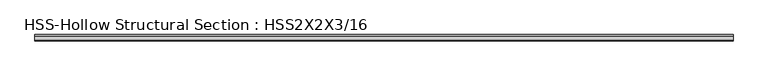
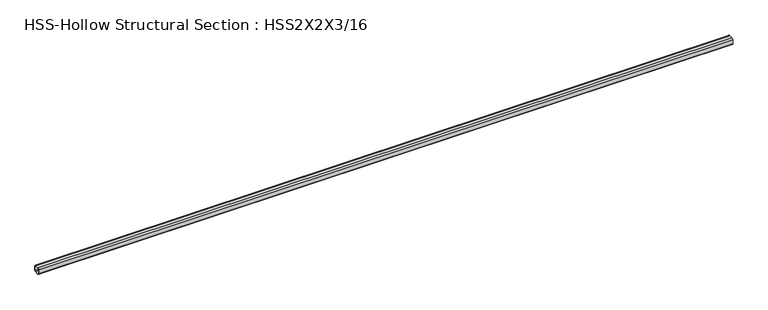
"""IFC4 building model written with IfcOpenShell, lengths in millimetres: beam geometry, HSS-Hollow Structural Section : HSS2X2X3/16."""

from ifc_helpers import new_model, si_unit, point, frame, frame_2d, origin, place, context, project, spatial, polyline, circle_curve, trimmed, segment, composite_curve, outline, extrude, source, transform, mapped, element, save


def hss_hollow_structural_section_hss2x2x3_16_21cd95f6(model_context):
    return source(origin(), model_context, "Body", "SweptSolid", [
        extrude(outline(composite_curve([segment(polyline([(25.4, 16.5608), (25.4, -16.5608)]), True, "CONTINUOUS"), segment(trimmed(circle_curve(frame_2d((16.5608, -16.5608)), 8.8392), [point((25.4, -16.5608))], [point((16.5608, -25.4))], False, "CARTESIAN"), True, "CONTINUOUS"), segment(polyline([(16.5608, -25.4), (-16.5608, -25.4)]), True, "CONTINUOUS"), segment(trimmed(circle_curve(frame_2d((-16.5608, -16.5608)), 8.8392), [point((-16.5608, -25.4))], [point((-25.4, -16.5608))], False, "CARTESIAN"), True, "CONTINUOUS"), segment(polyline([(-25.4, -16.5608), (-25.4, 16.5608)]), True, "CONTINUOUS"), segment(trimmed(circle_curve(frame_2d((-16.5608, 16.5608)), 8.8392), [point((-25.4, 16.5608))], [point((-16.5608, 25.4))], False, "CARTESIAN"), True, "CONTINUOUS"), segment(polyline([(-16.5608, 25.4), (16.5608, 25.4)]), True, "CONTINUOUS"), segment(trimmed(circle_curve(frame_2d((16.5608, 16.5608)), 8.8392), [point((16.5608, 25.4))], [point((25.4, 16.5608))], False, "CARTESIAN"), True, "CONTINUOUS")], self_intersect=False), holes=[composite_curve([segment(trimmed(circle_curve(frame_2d((-16.5608, 16.5608)), 4.4196), [point((-16.5608, 20.9804))], [point((-20.9804, 16.5608))], True, "CARTESIAN"), True, "CONTINUOUS"), segment(polyline([(-20.9804, 16.5608), (-20.9804, -16.5608)]), True, "CONTINUOUS"), segment(trimmed(circle_curve(frame_2d((-16.5608, -16.5608)), 4.4196), [point((-20.9804, -16.5608))], [point((-16.5608, -20.9804))], True, "CARTESIAN"), True, "CONTINUOUS"), segment(polyline([(-16.5608, -20.9804), (16.5608, -20.9804)]), True, "CONTINUOUS"), segment(trimmed(circle_curve(frame_2d((16.5608, -16.5608)), 4.4196), [point((16.5608, -20.9804))], [point((20.9804, -16.5608))], True, "CARTESIAN"), True, "CONTINUOUS"), segment(polyline([(20.9804, -16.5608), (20.9804, 16.5608)]), True, "CONTINUOUS"), segment(trimmed(circle_curve(frame_2d((16.5608, 16.5608)), 4.4196), [point((20.9804, 16.5608))], [point((16.5608, 20.9804))], True, "CARTESIAN"), True, "CONTINUOUS"), segment(polyline([(16.5608, 20.9804), (-16.5608, 20.9804)]), True, "CONTINUOUS")], self_intersect=False)]), frame((4003.675, 0.0, 0.0), z_axis=(1.0, 0.0, 0.0), x_axis=(0.0, 1.0, 0.0)), (0.0, 0.0, 1.0), 5458.61875),
    ])


if __name__ == "__main__":
    model = new_model("IFC4")
    model_context = context("Model", 3, world=origin())
    ifc_project = project(units=[si_unit("LENGTHUNIT", "METRE", prefix="MILLI")], contexts=[model_context])
    site = spatial("IfcSite", under=ifc_project)
    building = spatial("IfcBuilding", under=site)
    placement = place(None, origin())
    hss_hollow_structural_section_hss2x2x3_16_shape = hss_hollow_structural_section_hss2x2x3_16_21cd95f6(model_context)
    element("IfcBeam", 1, ObjectType="HSS-Hollow Structural Section : HSS2X2X3/16", at=placement, inside=building, context=model_context, shape_type="MappedRepresentation", body=[
        mapped(hss_hollow_structural_section_hss2x2x3_16_shape, transform((0.0, 0.0, 0.0), x_axis=(1.0, 0.0, 0.0), y_axis=(0.0, 1.0, 0.0), z_axis=(0.0, 0.0, 1.0))),
    ])
    save(model, "model.ifc")

# Revit data of these elements
# Type "HSS-Hollow Structural Section : HSS2X2X3/16"
#   Keynote = "M05121300.04"
#   Assembly Code = "B10"
#   Shape = "Square"
#   W = 4.3
#   Ht = 0' - 2"
#   Length [instance default] = 5' - 0"
#   b = 0' - 2"
#   kr = 0' - 0.348"
#   t = 0' - 0.174"
#   A = 0.00826389 SF
#   Structural Material [instance default] = Steel ASTM A500, Grade B, Rectangular and Square
# Element 1 (IfcBeam, "HSS-Hollow Structural Section : HSS2X2X3/16")
#   Materials on its faces: "Steel ASTM A500, Grade B, Rectangular and Square"
# Materials
#   "Steel ASTM A500, Grade B, Rectangular and Square": class "Metal", colour RGB 199 199 199, transparency 0, Description = "Carbon steel", Cost = 0
